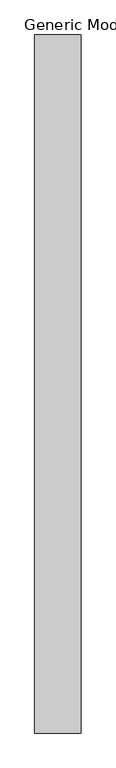
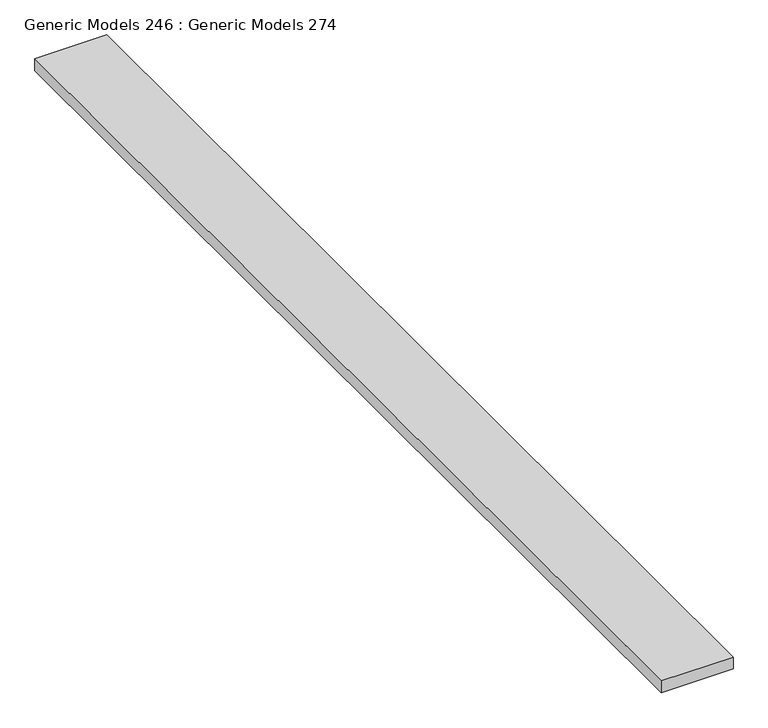
"""IFC4 building model written with IfcOpenShell, lengths in millimetres: proxy geometry, Generic Models 246 : Generic Models 274."""

from ifc_helpers import new_model, si_unit, origin, place, context, project, spatial, faceted_brep, source, transform, mapped, element, save


def generic_models_246_generic_models_274_74c46295(model_context):
    return source(origin(), model_context, "Body", "Brep", [
        faceted_brep([(32090.9670184, 39665.5833903, 266245.6765953), (32090.9670184, 39665.5833903, 266376.15), (32090.9670184, 28439.2747112, 266376.15), (32090.9670184, 28439.2747112, 266245.6765953), (32090.9670184, 39454.8946413, 266245.6765953), (31345.9673478, 39665.5833903, 266245.6765953), (31345.9673478, 28439.2747112, 266245.6765953), (31345.9673478, 28439.2747112, 266376.15), (31345.9673478, 39665.5833903, 266376.15)], [[[0, 1, 2, 3, 4]], [[5, 6, 7, 8]], [[3, 2, 7, 6]], [[0, 4, 3, 6, 5]], [[1, 0, 5, 8]], [[2, 1, 8, 7]]]),
    ])


if __name__ == "__main__":
    model = new_model("IFC4")
    model_context = context("Model", 3, world=origin())
    ifc_project = project(units=[si_unit("LENGTHUNIT", "METRE", prefix="MILLI")], contexts=[model_context])
    site = spatial("IfcSite", under=ifc_project)
    building = spatial("IfcBuilding", under=site)
    placement = place(None, origin())
    generic_models_246_generic_models_274_shape = generic_models_246_generic_models_274_74c46295(model_context)
    element("IfcBuildingElementProxy", 1, Name="Generic Models 246 : Generic Models 274", ObjectType="Generic Models 246 : Generic Models 274", at=placement, inside=building, context=model_context, shape_type="MappedRepresentation", body=[
        mapped(generic_models_246_generic_models_274_shape, transform((0.0, 0.0, 0.0), x_axis=(1.0, 0.0, 0.0), y_axis=(0.0, 1.0, 0.0), z_axis=(0.0, 0.0, 1.0))),
    ])
    save(model, "model.ifc")

# Revit data of these elements
# Element 1 (IfcBuildingElementProxy, "Generic Models 246 : Generic Models 274")
#   Materials on its faces: "CONCRETE SLAB"
# Materials
#   "CONCRETE SLAB": class "Concrete", colour RGB 192 192 192, transparency 0, Description = "Cast-in-place concrete", Cost = 0
